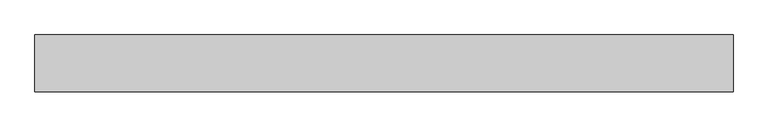
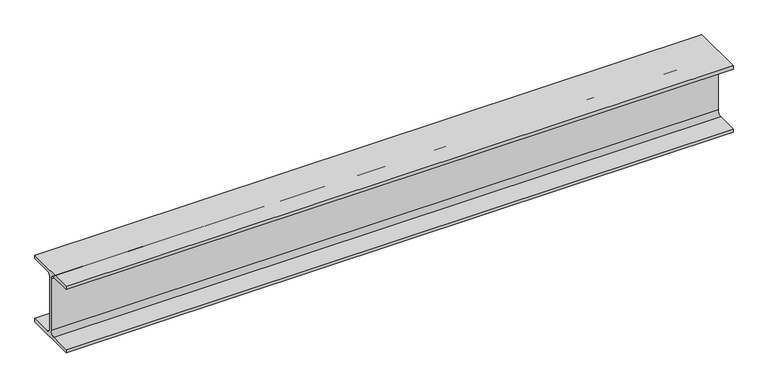
"""IFC4 building model written with IfcOpenShell, lengths in millimetres: beam geometry, 0912_Steel Framing_H-KSD3502 : H_SB_ASB_H-194x150x6x9."""

import ifcopenshell
import ifcopenshell.guid

model = None  # the IFC model being written
_history = None  # IfcOwnerHistory: only IFC2X3 demands one
_inside = {}  # id of a spatial element -> (the spatial element, [elements in it])
_under = {}  # id of a project, library or spatial element -> (it, [spatial elements below it])
_declared = {}  # id of a project -> (the project, [libraries it declares])
_typed = {}  # id of a type object -> (the type object, [elements of that type])
_made_of = {}  # id of a material, layer set ... -> (it, [elements and type objects made of it])


def new_model(schema):
    """Start an empty IFC model of exactly this schema.

    Asked for "IFC4X3", IfcOpenShell would pick the latest addendum, in which some entities
    have other attributes; the version numbers below select the first issue.
    IFC2X3 requires an IfcOwnerHistory on every rooted entity: one is made here for all.
    """
    global model, _history
    if schema == "IFC4X3":
        model = ifcopenshell.file(schema_version=(4, 3, 0, 0))
    else:
        model = ifcopenshell.file(schema=schema)
    _inside.clear()
    _under.clear()
    _declared.clear()
    _typed.clear()
    _made_of.clear()
    _history = None
    if model.schema == "IFC2X3":
        org = make("IfcOrganization", Name="unknown")
        user = make(
            "IfcPersonAndOrganization",
            ThePerson=make("IfcPerson", FamilyName="unknown"),
            TheOrganization=org,
        )
        app = make(
            "IfcApplication",
            ApplicationDeveloper=org,
            Version="unknown",
            ApplicationFullName="unknown",
            ApplicationIdentifier="unknown",
        )
        _history = make(
            "IfcOwnerHistory",
            OwningUser=user,
            OwningApplication=app,
            ChangeAction="ADDED",
            CreationDate=0,
        )
    return model


def make(cls, **values):
    """One entity of the class cls with the attributes given. An attribute that is None is left unset."""
    return model.create_entity(
        cls, **{name: value for name, value in values.items() if value is not None}
    )


def rooted(cls, **values):
    """An entity with a GlobalId (a new one), such as an element, a storey or a relation."""
    return make(cls, GlobalId=ifcopenshell.guid.new(), OwnerHistory=_history, **values)


def si_unit(unit_type, name, prefix=None):
    """IfcSIUnit, for example si_unit("LENGTHUNIT", "METRE", prefix="MILLI")."""
    return make("IfcSIUnit", UnitType=unit_type, Prefix=prefix, Name=name)


def assignment(units):
    """IfcUnitAssignment: the units of a project."""
    return None if units is None else make("IfcUnitAssignment", Units=units)


def point(xyz):
    """IfcCartesianPoint."""
    return None if xyz is None else make("IfcCartesianPoint", Coordinates=xyz)


def direction(xyz):
    """IfcDirection."""
    return None if xyz is None else make("IfcDirection", DirectionRatios=xyz)


def frame(location, z_axis=None, x_axis=None):
    """IfcAxis2Placement3D, a coordinate frame: its origin and axes. An axis left out is left unset."""
    return make(
        "IfcAxis2Placement3D",
        Location=point(location),
        Axis=direction(z_axis),
        RefDirection=direction(x_axis),
    )


def frame_2d(location, x_axis=None):
    """IfcAxis2Placement2D, a coordinate frame in the plane: its origin and x axis."""
    return make(
        "IfcAxis2Placement2D", Location=point(location), RefDirection=direction(x_axis)
    )


def origin():
    """The frame at (0, 0, 0) with its axes left unset."""
    return frame((0.0, 0.0, 0.0))


def place(relative_to, where):
    """IfcLocalPlacement: puts the frame where relative to a parent placement (None: the world)."""
    return make(
        "IfcLocalPlacement", PlacementRelTo=relative_to, RelativePlacement=where
    )


def context(
    kind, dimensions, precision=None, world=None, true_north=None, identifier=None
):
    """IfcGeometricRepresentationContext, for example the 3D "Model" context."""
    return make(
        "IfcGeometricRepresentationContext",
        ContextIdentifier=identifier,
        ContextType=kind,
        CoordinateSpaceDimension=dimensions,
        Precision=precision,
        WorldCoordinateSystem=world,
        TrueNorth=true_north,
    )


def project(units=None, contexts=None):
    """IfcProject with its units and contexts."""
    return rooted(
        "IfcProject",
        Name="project",
        RepresentationContexts=contexts,
        UnitsInContext=assignment(units),
    )


def spatial(cls, under=None, at=None, **own):
    """A site, building, storey or space (cls), placed at a placement, below another one or the project."""
    s = rooted(cls, ObjectPlacement=at, **own)
    if under is not None:
        _under.setdefault(under.id(), (under, []))[1].append(s)
    return s


def polyline(points):
    """IfcPolyline through the points."""
    return make("IfcPolyline", Points=[point(p) for p in points])


def circle_curve(where, radius):
    """IfcCircle in the frame where."""
    return make("IfcCircle", Position=where, Radius=radius)


def trimmed(basis, trim1, trim2, sense, master):
    """IfcTrimmedCurve: the piece of a basis curve between two trims."""
    return make(
        "IfcTrimmedCurve",
        BasisCurve=basis,
        Trim1=trim1,
        Trim2=trim2,
        SenseAgreement=sense,
        MasterRepresentation=master,
    )


def segment(curve, same_sense, transition):
    """IfcCompositeCurveSegment."""
    return make(
        "IfcCompositeCurveSegment",
        Transition=transition,
        SameSense=same_sense,
        ParentCurve=curve,
    )


def composite_curve(segments, self_intersect=None):
    """IfcCompositeCurve: segments joined end to end."""
    return make("IfcCompositeCurve", Segments=segments, SelfIntersect=self_intersect)


def outline(outer, holes=None, kind="AREA"):
    """IfcArbitraryClosedProfileDef: a profile drawn as a closed curve; with holes, ...WithVoids."""
    if holes is None:
        return make("IfcArbitraryClosedProfileDef", ProfileType=kind, OuterCurve=outer)
    return make(
        "IfcArbitraryProfileDefWithVoids",
        ProfileType=kind,
        OuterCurve=outer,
        InnerCurves=holes,
    )


def extrude(swept, where, along, depth):
    """IfcExtrudedAreaSolid: the profile swept, set in the frame where, extruded along a direction by depth."""
    return make(
        "IfcExtrudedAreaSolid",
        SweptArea=swept,
        Position=where,
        ExtrudedDirection=direction(along),
        Depth=depth,
    )


def shape(context_of_items, identifier, shape_type, items):
    """IfcShapeRepresentation: the items that make up one representation, for example the "Body"."""
    return make(
        "IfcShapeRepresentation",
        ContextOfItems=context_of_items,
        RepresentationIdentifier=identifier,
        RepresentationType=shape_type,
        Items=items,
    )


def source(mapping_origin, context_of_items, identifier, shape_type, items):
    """IfcRepresentationMap: a shape defined once, which mapped items show again and again."""
    return make(
        "IfcRepresentationMap",
        MappingOrigin=mapping_origin,
        MappedRepresentation=shape(context_of_items, identifier, shape_type, items),
    )


def transform(
    local_origin,
    x_axis=None,
    y_axis=None,
    z_axis=None,
    scale=None,
    scale2=None,
    scale3=None,
    uniform=True,
):
    """IfcCartesianTransformationOperator3D, or its non-uniform kind. x_axis, y_axis, z_axis: its Axis1, 2, 3."""
    if uniform:
        return make(
            "IfcCartesianTransformationOperator3D",
            Axis1=direction(x_axis),
            Axis2=direction(y_axis),
            LocalOrigin=point(local_origin),
            Scale=scale,
            Axis3=direction(z_axis),
        )
    return make(
        "IfcCartesianTransformationOperator3DnonUniform",
        Axis1=direction(x_axis),
        Axis2=direction(y_axis),
        LocalOrigin=point(local_origin),
        Scale=scale,
        Axis3=direction(z_axis),
        Scale2=scale2,
        Scale3=scale3,
    )


def mapped(mapping_source, mapping_target):
    """IfcMappedItem: shows the shape of a source again, moved by a transform."""
    return make(
        "IfcMappedItem", MappingSource=mapping_source, MappingTarget=mapping_target
    )


def made_of(thing, what):
    """Note that an element or type object is made of a material, layer set ...; save() writes the relation."""
    if what is not None:
        _made_of.setdefault(what.id(), (what, []))[1].append(thing)
    return thing


def element(
    cls,
    number,
    at=None,
    inside=None,
    cuts=None,
    type_object=None,
    material=None,
    context=None,
    identifier="Body",
    shape_type=None,
    held_by="IfcProductDefinitionShape",
    body=None,
    shapes=None,
    **own,
):
    """One element of the class cls, such as IfcWall. Its Tag is "e" and its number.

    at: its placement. inside: the storey or other place that contains it. cuts: it is an
    opening in that element (IfcRelVoidsElement). A single representation is given by context,
    identifier, shape_type and body (its items); several are given by shapes. held_by: the class
    of the entity that holds the representations. save() writes the other relations.
    """
    e = rooted(cls, Tag="e%d" % number, ObjectPlacement=at, **own)
    if body is not None:
        shapes = [shape(context, identifier, shape_type, body)]
    if shapes is not None:
        e.Representation = make(held_by, Representations=shapes)
    if inside is not None:
        _inside.setdefault(inside.id(), (inside, []))[1].append(e)
    if cuts is not None:
        rooted(
            "IfcRelVoidsElement", RelatingBuildingElement=cuts, RelatedOpeningElement=e
        )
    if type_object is not None:
        _typed.setdefault(type_object.id(), (type_object, []))[1].append(e)
    return made_of(e, material)


def aggregate(whole, parts):
    """IfcRelAggregates: a whole, such as a stair, and the parts it consists of."""
    return rooted("IfcRelAggregates", RelatingObject=whole, RelatedObjects=parts)


def save(model, path):
    """Write the relations noted so far, then the file.

    IfcRelAggregates (storeys below a building ...), IfcRelContainedInSpatialStructure (elements
    in a storey), IfcRelDefinesByType, IfcRelAssociatesMaterial and IfcRelDeclares: one each for
    every whole, place, type object, material and project.
    """
    for whole, parts in _under.values():
        aggregate(whole, parts)
    for where, things in _inside.values():
        rooted(
            "IfcRelContainedInSpatialStructure",
            RelatedElements=things,
            RelatingStructure=where,
        )
    for kind, things in _typed.values():
        rooted("IfcRelDefinesByType", RelatedObjects=things, RelatingType=kind)
    for what, things in _made_of.values():
        rooted("IfcRelAssociatesMaterial", RelatedObjects=things, RelatingMaterial=what)
    for by, libraries in _declared.values():
        rooted("IfcRelDeclares", RelatingContext=by, RelatedDefinitions=libraries)
    model.write(path)


def beam_b633f717(model_context):
    return source(origin(), model_context, "Body", "SweptSolid", [
        extrude(outline(composite_curve([segment(polyline([(75.0, -88.0), (75.0, -97.0), (-75.0, -97.0), (-75.0, -88.0), (-16.0, -88.0)]), True, "CONTINUOUS"), segment(trimmed(circle_curve(frame_2d((-16.0, -75.0)), 13.0), [point((-16.0, -88.0))], [point((-3.0, -75.0))], True, "CARTESIAN"), True, "CONTINUOUS"), segment(polyline([(-3.0, -75.0), (-3.0, 75.0)]), True, "CONTINUOUS"), segment(trimmed(circle_curve(frame_2d((-16.0, 75.0)), 13.0), [point((-3.0, 75.0))], [point((-16.0, 88.0))], True, "CARTESIAN"), True, "CONTINUOUS"), segment(polyline([(-16.0, 88.0), (-75.0, 88.0), (-75.0, 97.0), (75.0, 97.0), (75.0, 88.0), (16.0, 88.0)]), True, "CONTINUOUS"), segment(trimmed(circle_curve(frame_2d((16.0, 75.0)), 13.0), [point((16.0, 88.0))], [point((3.0, 75.0))], True, "CARTESIAN"), True, "CONTINUOUS"), segment(polyline([(3.0, 75.0), (3.0, -75.0)]), True, "CONTINUOUS"), segment(trimmed(circle_curve(frame_2d((16.0, -75.0)), 13.0), [point((3.0, -75.0))], [point((16.0, -88.0))], True, "CARTESIAN"), True, "CONTINUOUS"), segment(polyline([(16.0, -88.0), (75.0, -88.0)]), True, "CONTINUOUS")], self_intersect=False)), frame((-853.4240734, 0.0, 0.0), z_axis=(1.0, 0.0, 0.0), x_axis=(0.0, 1.0, 0.0)), (0.0, 0.0, 1.0), 1846.5746098),
    ])


if __name__ == "__main__":
    model = new_model("IFC4")
    model_context = context("Model", 3, world=origin())
    ifc_project = project(units=[si_unit("LENGTHUNIT", "METRE", prefix="MILLI")], contexts=[model_context])
    site = spatial("IfcSite", under=ifc_project)
    building = spatial("IfcBuilding", under=site)
    placement = place(None, origin())
    beam_shape = beam_b633f717(model_context)
    element("IfcBeam", 1, ObjectType="0912_Steel Framing_H-KSD3502 : H_SB_ASB_H-194x150x6x9", at=placement, inside=building, context=model_context, shape_type="MappedRepresentation", body=[
        mapped(beam_shape, transform((0.0, 0.0, 0.0), x_axis=(1.0, 0.0, 0.0), y_axis=(0.0, 1.0, 0.0), z_axis=(0.0, 0.0, 1.0))),
    ])
    save(model, "model.ifc")

# Revit data of these elements
# Type "0912_Steel Framing_H-KSD3502 : H_SB_ASB_H-194x150x6x9"
#   H_WM Code_1 = "S01AA002-00001 | Main Steel Structure Fabrication Work | Shelter/Building | Medium Steel - Standard (90KG/M>Weight≥30KG/M) | Material: (   )"
#   H_WM Code_2 = "S03AA028-00001 | Main Steel Structure Erection Work | Shelter/Building | Medium Steel (90KG/M>Weight≥30KG/M) | Material: (   )"
#   H_WM Code_3 = "S01AA010-00001 | Main Steel Structure Fabrication Work | Shelter/Building | Steel Painting/Coating | for Non-Fireproofed Steel Surface, Surface Preparation, Primer, Second & Final Coat | Material: (   )"
#   H_Q'ty Cal Type Tag = "SB-Q2"
#   Width = 15.0 cm
#   Web Thickness = 0.6 cm
#   Web Fillet = 1.3 cm
#   Warping Constant = 43316.0 cm⁶
#   W = 0
#   Torsional Moment of Inertia = 8.622 cm⁴
#   Section Area = 39.01 cm²
#   Plastic Modulus weak axis = 104.0 cm³
#   Plastic Modulus strong axis = 309.0 cm³
#   Perimeter = 0.95 m²/m
#   Nominal Weight = 30.60 kgf/m
#   Moment of Inertia weak axis = 507.00 cm⁴
#   Moment of Inertia strong axis = 2690.00 cm⁴
#   Height = 19.4 cm
#   Flange Thickness = 0.9 cm
#   Elastic Modulus weak axis = 67.6 cm³
#   Elastic Modulus strong axis = 277.0 cm³
#   Centroid Vertical = 9.7 cm
#   Centroid Horizontal = 7.5 cm
#   Ix = 26900000
#   Length [instance default] = 1.5240 m
#   Zx = 309000
#   b = 0.1500 m
#   h = 0.1940 m
#   r = 0.0130 m
#   s = 0.0060 m
#   t = 0.0090 m
#   A = 0.003901 m²
#   Structural Material [instance default] = Steel, 45-345
#   Assembly Code = ""
# Element 1 (IfcBeam, "0912_Steel Framing_H-KSD3502 : H_SB_ASB_H-194x150x6x9")
#   Structural Material = none
# Materials
#   "Steel, 45-345": class "Metal", colour RGB 189 187 185, transparency 0, Description = "Steel 345 MPa", Cost = 0
